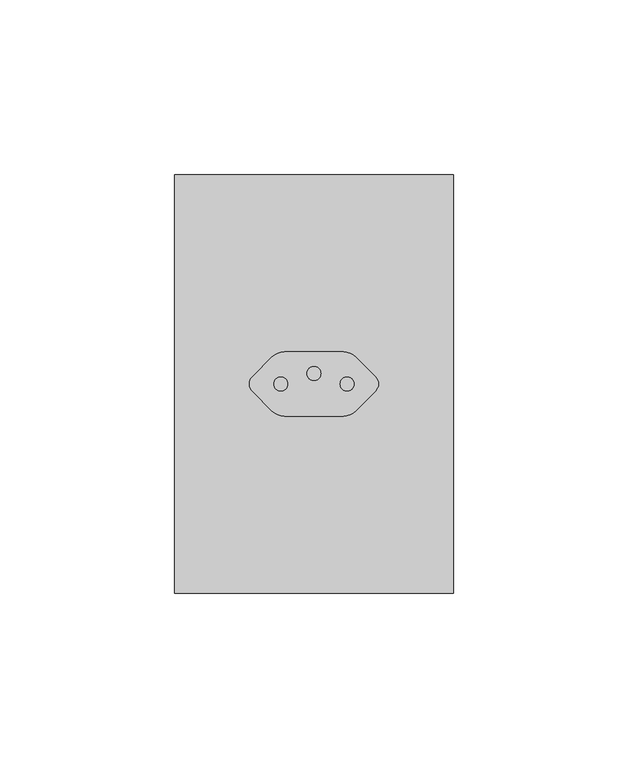
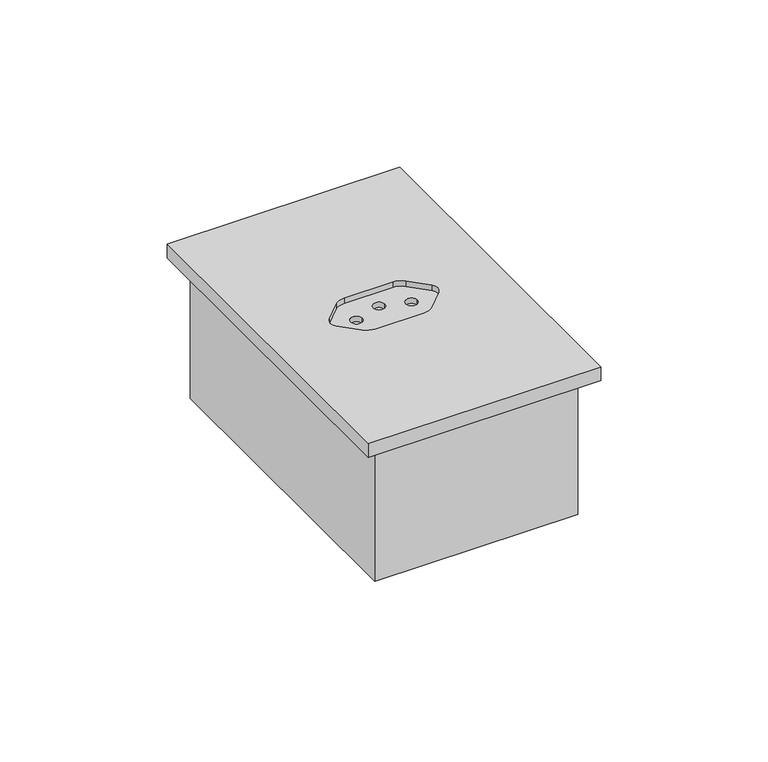
"""IFC4 building model written with IfcOpenShell, lengths in millimetres: proxy geometry, CAIXA VERTICE V7 : Tomada 10A 1s."""

from ifc_helpers import new_model, si_unit, frame, origin, place, context, project, spatial, polyline, circle_curve, faceted_brep, source, transform, mapped, element, save
from ifc_brep_helpers import plane_surface, revolved_surface, advanced_brep


def electrical_fixtures_759cbdb1(model_context):
    return source(origin(), model_context, "Body", "SolidModel", [
        faceted_brep([(35.0, 1155.0, 0.0), (-35.0, 1155.0, 0.0), (-35.0, 1045.0, 0.0), (35.0, 1045.0, 0.0), (33.0, 1153.0, 0.0), (33.0, 1047.0, 0.0), (-33.0, 1047.0, 0.0), (-33.0, 1153.0, 0.0), (33.0, 1047.0, -48.0), (33.0, 1153.0, -48.0), (-33.0, 1153.0, -48.0), (-33.0, 1047.0, -48.0), (35.0, 1155.0, -50.0), (35.0, 1045.0, -50.0), (-35.0, 1045.0, -50.0), (-35.0, 1155.0, -50.0)], [[[0, 1, 2, 3], [4, 5, 6, 7]], [[8, 9, 10, 11]], [[12, 13, 14, 15]], [[12, 15, 1, 0]], [[1, 15, 14, 2]], [[2, 14, 13, 3]], [[3, 13, 12, 0]], [[5, 4, 9, 8]], [[6, 5, 8, 11]], [[7, 6, 11, 10]], [[4, 7, 10, 9]]]),
        advanced_brep(
        [(40.0, 1160.0, 5.0), (-40.0, 1160.0, 5.0), (-40.0, 1040.0, 5.0), (40.0, 1040.0, 5.0), (8.4215729, 1090.75, 5.0), (-8.4215729, 1090.75, 5.0), (-11.9571068, 1092.2144661, 5.0), (-17.6213203, 1097.8786797, 5.0), (-17.6213203, 1102.1213203, 5.0), (-11.9571068, 1107.7855339, 5.0), (-8.4215729, 1109.25, 5.0), (8.4215729, 1109.25, 5.0), (11.9571068, 1107.7855339, 5.0), (17.6213203, 1102.1213203, 5.0), (17.6213203, 1097.8786797, 5.0), (11.9571068, 1092.2144661, 5.0), (-40.0, 1160.0, 0.0), (40.0, 1160.0, 0.0), (40.0, 1040.0, 0.0), (-40.0, 1040.0, 0.0), (8.4215729, 1090.75, 3.0), (11.9571068, 1092.2144661, 3.0), (17.6213203, 1097.8786797, 3.0), (17.6213203, 1102.1213203, 3.0), (11.9571068, 1107.7855339, 3.0), (8.4215729, 1109.25, 3.0), (-8.4215729, 1109.25, 3.0), (-11.9571068, 1107.7855339, 3.0), (-17.6213203, 1102.1213203, 3.0), (-17.6213203, 1097.8786797, 3.0), (-11.9571068, 1092.2144661, 3.0), (-8.4215729, 1090.75, 3.0), (-7.5, 1100.0, 3.0), (-11.5, 1100.0, 3.0), (11.5, 1100.0, 3.0), (7.5, 1100.0, 3.0), (2.0, 1103.0, 3.0), (-2.0, 1103.0, 3.0), (-11.5, 1100.0, 1.0), (-7.5, 1100.0, 1.0), (7.5, 1100.0, 1.0), (11.5, 1100.0, 1.0), (-2.0, 1103.0, 1.0), (2.0, 1103.0, 1.0)],
        [
            (0, 1),
            (1, 2),
            (2, 3),
            (3, 0),
            (4, 5),
            (5, 6, circle_curve(frame((-8.4215729, 1095.75, 5.0), z_axis=(0.0, 0.0, -1.0), x_axis=(-1.0, 0.0, 0.0)), 5.0)),
            (6, 7),
            (7, 8, circle_curve(frame((-15.5, 1100.0, 5.0), z_axis=(0.0, 0.0, -1.0), x_axis=(-1.0, 0.0, 0.0)), 3.0)),
            (8, 9),
            (9, 10, circle_curve(frame((-8.4215729, 1104.25, 5.0), z_axis=(0.0, 0.0, -1.0), x_axis=(-1.0, 0.0, 0.0)), 5.0)),
            (10, 11),
            (11, 12, circle_curve(frame((8.4215729, 1104.25, 5.0), z_axis=(0.0, 0.0, -1.0), x_axis=(-1.0, 0.0, 0.0)), 5.0)),
            (12, 13),
            (13, 14, circle_curve(frame((15.5, 1100.0, 5.0), z_axis=(0.0, 0.0, -1.0), x_axis=(-1.0, 0.0, 0.0)), 3.0)),
            (14, 15),
            (15, 4, circle_curve(frame((8.4215729, 1095.75, 5.0), z_axis=(0.0, 0.0, -1.0), x_axis=(-1.0, 0.0, 0.0)), 5.0)),
            (16, 17),
            (17, 18),
            (18, 19),
            (19, 16),
            (0, 17),
            (16, 1),
            (19, 2),
            (18, 3),
            (20, 21, circle_curve(frame((8.4215729, 1095.75, 3.0), z_axis=(0.0, 0.0, 1.0), x_axis=(-1.0, 0.0, 0.0)), 5.0)),
            (21, 22),
            (22, 23, circle_curve(frame((15.5, 1100.0, 3.0), z_axis=(0.0, 0.0, 1.0), x_axis=(-1.0, 0.0, 0.0)), 3.0)),
            (23, 24),
            (24, 25, circle_curve(frame((8.4215729, 1104.25, 3.0), z_axis=(0.0, 0.0, 1.0), x_axis=(-1.0, 0.0, 0.0)), 5.0)),
            (25, 26),
            (26, 27, circle_curve(frame((-8.4215729, 1104.25, 3.0), z_axis=(0.0, 0.0, 1.0), x_axis=(-1.0, 0.0, 0.0)), 5.0)),
            (27, 28),
            (28, 29, circle_curve(frame((-15.5, 1100.0, 3.0), z_axis=(0.0, 0.0, 1.0), x_axis=(-1.0, 0.0, 0.0)), 3.0)),
            (29, 30),
            (30, 31, circle_curve(frame((-8.4215729, 1095.75, 3.0), z_axis=(0.0, 0.0, 1.0), x_axis=(-1.0, 0.0, 0.0)), 5.0)),
            (31, 20),
            (32, 33, circle_curve(frame((-9.5, 1100.0, 3.0), z_axis=(0.0, 0.0, -1.0), x_axis=(1.0, 2.301812013077709e-12, 0.0)), 2.0)),
            (33, 32, circle_curve(frame((-9.5, 1100.0, 3.0), z_axis=(0.0, 0.0, -1.0), x_axis=(1.0, 2.301812013077709e-12, 0.0)), 2.0)),
            (34, 35, circle_curve(frame((9.5, 1100.0, 3.0), z_axis=(0.0, 0.0, -1.0), x_axis=(1.0, 2.301812013077709e-12, 0.0)), 2.0)),
            (35, 34, circle_curve(frame((9.5, 1100.0, 3.0), z_axis=(0.0, 0.0, -1.0), x_axis=(1.0, 2.301812013077709e-12, 0.0)), 2.0)),
            (36, 37, circle_curve(frame((0.0, 1103.0, 3.0), z_axis=(0.0, 0.0, -1.0), x_axis=(1.0, 2.301812013077709e-12, 0.0)), 2.0)),
            (37, 36, circle_curve(frame((0.0, 1103.0, 3.0), z_axis=(0.0, 0.0, -1.0), x_axis=(1.0, 2.301812013077709e-12, 0.0)), 2.0)),
            (31, 5),
            (4, 20),
            (30, 6),
            (29, 7),
            (28, 8),
            (27, 9),
            (26, 10),
            (25, 11),
            (24, 12),
            (23, 13),
            (22, 14),
            (21, 15),
            (38, 39, circle_curve(frame((-9.5, 1100.0, 1.0), z_axis=(0.0, 0.0, 1.0), x_axis=(1.0, 2.301812013077709e-12, 0.0)), 2.0)),
            (39, 38, circle_curve(frame((-9.5, 1100.0, 1.0), z_axis=(0.0, 0.0, 1.0), x_axis=(1.0, 2.301812013077709e-12, 0.0)), 2.0)),
            (40, 41, circle_curve(frame((9.5, 1100.0, 1.0), z_axis=(0.0, 0.0, 1.0), x_axis=(1.0, 2.301812013077709e-12, 0.0)), 2.0)),
            (41, 40, circle_curve(frame((9.5, 1100.0, 1.0), z_axis=(0.0, 0.0, 1.0), x_axis=(1.0, 2.301812013077709e-12, 0.0)), 2.0)),
            (42, 43, circle_curve(frame((0.0, 1103.0, 1.0), z_axis=(0.0, 0.0, 1.0), x_axis=(1.0, 2.301812013077709e-12, 0.0)), 2.0)),
            (43, 42, circle_curve(frame((0.0, 1103.0, 1.0), z_axis=(0.0, 0.0, 1.0), x_axis=(1.0, 2.301812013077709e-12, 0.0)), 2.0)),
            (32, 39),
            (38, 33),
            (34, 41),
            (40, 35),
            (36, 43),
            (42, 37),
        ],
        [
            plane_surface(frame((-60.0, 1160.0, 5.0), z_axis=(0.0, 0.0, 1.0), x_axis=(-1.0, 0.0, 0.0))),
            plane_surface(frame((-60.0, 1160.0, 0.0), z_axis=(0.0, 0.0, -1.0), x_axis=(1.0, 0.0, 0.0))),
            plane_surface(frame((40.0, 1160.0, 5.0), z_axis=(0.0, 1.0, 0.0), x_axis=(0.0, 0.0, -1.0))),
            plane_surface(frame((-40.0, 1160.0, 5.0), z_axis=(-1.0, 0.0, 0.0), x_axis=(0.0, 0.0, -1.0))),
            plane_surface(frame((-40.0, 1040.0, 5.0), z_axis=(0.0, -1.0, 0.0), x_axis=(0.0, 0.0, -1.0))),
            plane_surface(frame((40.0, 1040.0, 5.0), z_axis=(1.0, 0.0, 0.0), x_axis=(0.0, 0.0, -1.0))),
            plane_surface(frame((3.4215729, 1095.75, 3.0), z_axis=(0.0, 0.0, 1.0), x_axis=(0.0, 1.0, 0.0))),
            plane_surface(frame((-8.4215729, 1090.75, 5.0), z_axis=(0.0, 1.0, 0.0), x_axis=(0.0, 0.0, -1.0))),
            revolved_surface(polyline([(-13.4215729, 1095.75, 5.0), (-13.4215729, 1095.75, 3.0)]), (-8.4215729, 1095.75, 3.0), (0.0, 0.0, 1.0)),
            plane_surface(frame((-17.6213203, 1097.8786797, 5.0), z_axis=(0.7071067811865045, 0.7071067811865905, 0.0), x_axis=(0.0, 0.0, -1.0))),
            revolved_surface(polyline([(-18.5, 1100.0, 5.0), (-18.5, 1100.0, 3.0)]), (-15.5, 1100.0, 3.0), (0.0, 0.0, 1.0)),
            plane_surface(frame((-11.9571068, 1107.7855339, 5.0), z_axis=(0.7071067811865515, -0.7071067811865437, 0.0), x_axis=(0.0, 0.0, -1.0))),
            revolved_surface(polyline([(-13.4215729, 1104.25, 5.0), (-13.4215729, 1104.25, 3.0)]), (-8.4215729, 1104.25, 3.0), (0.0, 0.0, 1.0)),
            plane_surface(frame((8.4215729, 1109.25, 5.0), z_axis=(0.0, -1.0, 0.0), x_axis=(0.0, 0.0, -1.0))),
            revolved_surface(polyline([(3.4215728999999993, 1104.25, 5.0), (3.4215728999999993, 1104.25, 3.0)]), (8.4215729, 1104.25, 3.0), (0.0, 0.0, 1.0)),
            plane_surface(frame((17.6213203, 1102.1213203, 5.0), z_axis=(-0.7071067811865307, -0.7071067811865643, 0.0), x_axis=(0.0, 0.0, -1.0))),
            revolved_surface(polyline([(12.5, 1100.0, 5.0), (12.5, 1100.0, 3.0)]), (15.5, 1100.0, 3.0), (0.0, 0.0, 1.0)),
            plane_surface(frame((11.9571068, 1092.2144661, 5.0), z_axis=(-0.7071067811865893, 0.7071067811865058, 0.0), x_axis=(0.0, 0.0, -1.0))),
            revolved_surface(polyline([(3.4215728999999993, 1095.75, 5.0), (3.4215728999999993, 1095.75, 3.0)]), (8.4215729, 1095.75, 3.0), (0.0, 0.0, 1.0)),
            plane_surface(frame((-7.5, 1100.0, 1.0), z_axis=(0.0, 0.0, 1.0), x_axis=(2.301812013077709e-12, -1.0, 0.0))),
            revolved_surface(polyline([(-7.5, 1100.0000000000045, 3.0), (-7.5, 1100.0000000000045, 1.0)]), (-9.5, 1100.0, 1.0), (0.0, 0.0, 1.0)),
            revolved_surface(polyline([(11.5, 1100.0000000000045, 3.0), (11.5, 1100.0000000000045, 1.0)]), (9.5, 1100.0, 5.0), (0.0, 0.0, 1.0)),
            revolved_surface(polyline([(2.0, 1103.0000000000045, 3.0), (2.0, 1103.0000000000045, 1.0)]), (0.0, 1103.0, 5.0), (0.0, 0.0, 1.0)),
        ],
        [
            (0, [[1, 2, 3, 4], [5, 6, 7, 8, 9, 10, 11, 12, 13, 14, 15, 16]]),
            (1, [[17, 18, 19, 20]]),
            (2, [[-1, 21, -17, 22]]),
            (3, [[-2, -22, -20, 23]]),
            (4, [[-3, -23, -19, 24]]),
            (5, [[-4, -24, -18, -21]]),
            (6, [[25, 26, 27, 28, 29, 30, 31, 32, 33, 34, 35, 36], [37, 38], [39, 40], [41, 42]]),
            (7, [[-36, 43, -5, 44]]),
            (8, [[-35, 45, -6, -43]]),
            (9, [[-34, 46, -7, -45]]),
            (10, [[-33, 47, -8, -46]]),
            (11, [[-32, 48, -9, -47]]),
            (12, [[-31, 49, -10, -48]]),
            (13, [[-30, 50, -11, -49]]),
            (14, [[-29, 51, -12, -50]]),
            (15, [[-28, 52, -13, -51]]),
            (16, [[-27, 53, -14, -52]]),
            (17, [[-26, 54, -15, -53]]),
            (18, [[-25, -44, -16, -54]]),
            (19, [[55, 56]]),
            (19, [[57, 58]]),
            (19, [[59, 60]]),
            (20, [[-37, 61, -55, 62]]),
            (20, [[-38, -62, -56, -61]]),
            (21, [[-39, 63, -57, 64]]),
            (21, [[-40, -64, -58, -63]]),
            (22, [[-41, 65, -59, 66]]),
            (22, [[-42, -66, -60, -65]]),
        ],
    ),
    ])


if __name__ == "__main__":
    model = new_model("IFC4")
    model_context = context("Model", 3, world=origin())
    ifc_project = project(units=[si_unit("LENGTHUNIT", "METRE", prefix="MILLI")], contexts=[model_context])
    site = spatial("IfcSite", under=ifc_project)
    building = spatial("IfcBuilding", under=site)
    placement = place(None, origin())
    electrical_fixtures_shape = electrical_fixtures_759cbdb1(model_context)
    element("IfcBuildingElementProxy", 1, Name="CAIXA VERTICE V7 : Tomada 10A 1s", ObjectType="CAIXA VERTICE V7 : Tomada 10A 1s", at=placement, inside=building, context=model_context, shape_type="MappedRepresentation", body=[
        mapped(electrical_fixtures_shape, transform((0.0, 0.0, 0.0), x_axis=(1.0, 0.0, 0.0), y_axis=(0.0, 1.0, 0.0), z_axis=(0.0, 0.0, 1.0))),
    ])
    save(model, "model.ifc")

# Revit data of these elements
# Type "CAIXA VERTICE V7 : Tomada 10A 1s"
#   URL = "www.facebook.com/verticetreinamentos"
#   SEÇÃO [instance default] = ""
#   Rotação [instance default] = 0.00°
#   LARGURA DA TAMPA = 0.08 m
#   BORDA = 0.01 m
#   ALTURA DE INSTALAÇÃO [instance default] = 1.10 m
#   Distância Anotação [instance default] = 0.0015 m
#   ALTURA DA TAMPA = 0.12 m
#   Vertical [instance default] = yes
#   VER SEÇÃO [instance default] = no
#   SHADE ESQ [instance default] = no
#   SHADE DIR [instance default] = yes
#   HORIZONTAL [instance default] = no
#   ANDAR COM A LEGENDA [instance default] = 0
#   Material Tampa [instance default] = Plástico, branco opaco
#   Caixa = element 1798514
#   Anotação = element 1798528
#   Default Elevation = 0
# Element 1 (IfcBuildingElementProxy, "CAIXA VERTICE V7 : Tomada 10A 1s")
#   Materials on its faces: "Plástico, branco opaco"
# Materials
#   "Plástico, branco opaco": class "Plástico", colour RGB 120 120 120, transparency 0, Description = "Plastic, generic, opaque white", Cost = 0
